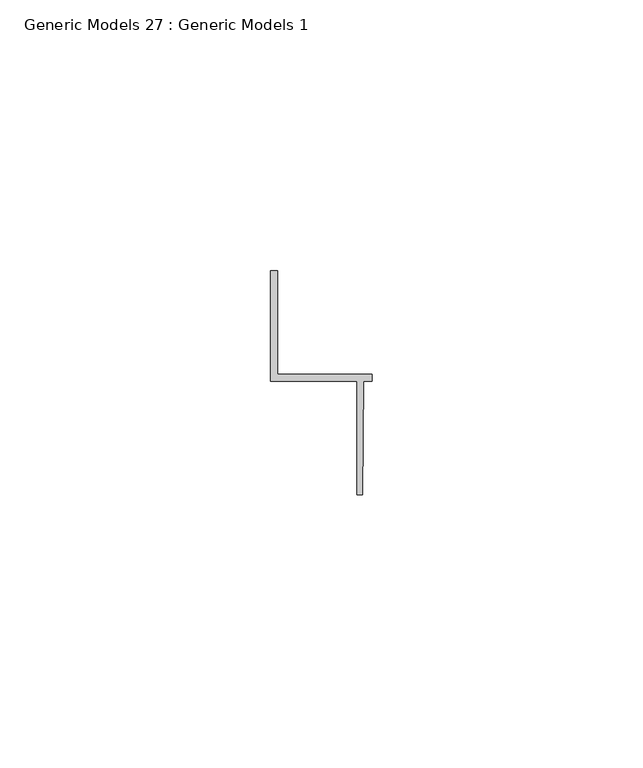
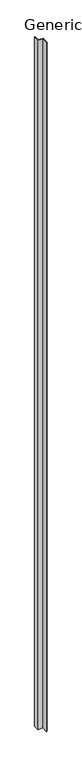
"""IFC4 building model written with IfcOpenShell, lengths in millimetres: proxy geometry, Generic Models 27 : Generic Models 1."""

from ifc_helpers import new_model, si_unit, frame, origin, place, context, project, spatial, polyline, outline, extrude, source, transform, mapped, element, save


def generic_models_27_generic_models_1_181a5866(model_context):
    return source(origin(), model_context, "Body", "SweptSolid", [
        extrude(outline(polyline([(14516.7945817, 5560.0067134), (14515.2705817, 5560.0067134), (14515.0103115, 5539.0517232), (14514.0005817, 5539.0517232), (14514.0005817, 5560.0067134), (14498.1255817, 5560.0067134), (14498.1255817, 5580.3267134), (14499.3955817, 5580.3267134), (14499.3955817, 5561.2767134), (14516.7945817, 5561.2767134), (14516.7945817, 5560.0067134)])), frame((0.0, 0.0, 450.7860265), z_axis=(0.0, 0.0, 1.0), x_axis=(1.0, 0.0, 0.0)), (0.0, 0.0, 1.0), 2444.75),
    ])


if __name__ == "__main__":
    model = new_model("IFC4")
    model_context = context("Model", 3, world=origin())
    ifc_project = project(units=[si_unit("LENGTHUNIT", "METRE", prefix="MILLI")], contexts=[model_context])
    site = spatial("IfcSite", under=ifc_project)
    building = spatial("IfcBuilding", under=site)
    placement = place(None, origin())
    generic_models_27_generic_models_1_shape = generic_models_27_generic_models_1_181a5866(model_context)
    element("IfcBuildingElementProxy", 1, Name="Generic Models 27 : Generic Models 1", ObjectType="Generic Models 27 : Generic Models 1", at=placement, inside=building, context=model_context, shape_type="MappedRepresentation", body=[
        mapped(generic_models_27_generic_models_1_shape, transform((0.0, 0.0, 0.0), x_axis=(1.0, 0.0, 0.0), y_axis=(0.0, 1.0, 0.0), z_axis=(0.0, 0.0, 1.0))),
    ])
    save(model, "model.ifc")

# Revit data of these elements
# Element 1 (IfcBuildingElementProxy, "Generic Models 27 : Generic Models 1")
#   Materials on its faces: "ALUM. HEADER PROFILE TO MATCH EXISTING AT TENANT ENTRANCE"
# Materials
#   "ALUM. HEADER PROFILE TO MATCH EXISTING AT TENANT ENTRANCE": class "Unassigned", colour RGB 226 225 224, transparency 0, Cost = 0
